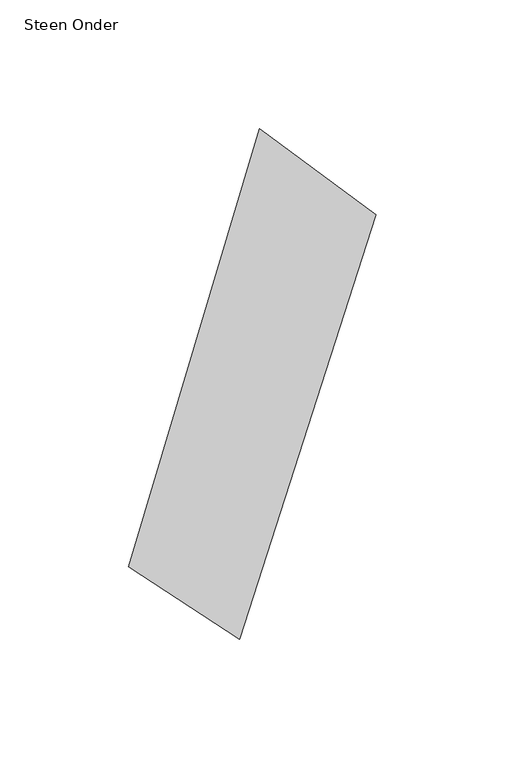
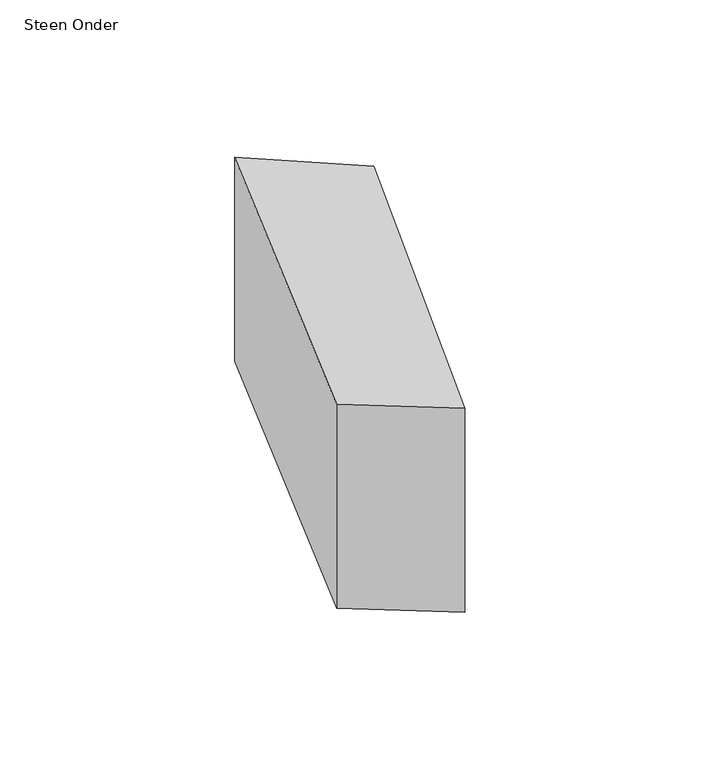
"""IFC4 building model written with IfcOpenShell, lengths in millimetres: proxy geometry, 00_GMA_steen_versie_4 : Steen Onder."""

from ifc_helpers import new_model, si_unit, origin, origin_with_axes, place, context, project, spatial, polyline, outline, extrude, source, transform, mapped, element, save


def steen_onder_082d7394(model_context):
    return source(origin(), model_context, "Body", "SweptSolid", [
        extrude(outline(polyline([(127.1998876, 151.3789965), (74.2256796, -13.1550493), (31.2595891, 14.8619373), (82.1091375, 184.7796986), (127.1998876, 151.3789965)])), origin_with_axes(), (0.0, 0.0, 1.0), 100.0),
    ])


if __name__ == "__main__":
    model = new_model("IFC4")
    model_context = context("Model", 3, world=origin())
    ifc_project = project(units=[si_unit("LENGTHUNIT", "METRE", prefix="MILLI")], contexts=[model_context])
    site = spatial("IfcSite", under=ifc_project)
    building = spatial("IfcBuilding", under=site)
    placement = place(None, origin())
    steen_onder_shape = steen_onder_082d7394(model_context)
    element("IfcBuildingElementProxy", 1, Name="00_GMA_steen_versie_4 : Steen Onder", ObjectType="00_GMA_steen_versie_4 : Steen Onder", at=placement, inside=building, context=model_context, shape_type="MappedRepresentation", body=[
        mapped(steen_onder_shape, transform((0.0, 0.0, 0.0), x_axis=(1.0, 0.0, 0.0), y_axis=(0.0, 1.0, 0.0), z_axis=(0.0, 0.0, 1.0))),
    ])
    save(model, "model.ifc")

# Revit data of these elements
# Type "00_GMA_steen_versie_4 : Steen Onder"
#   StootVoegHalfBoven [instance default] = 5 mm
#   StootVoegHalf [instance default] = 5 mm
#   StootVoegBreedteOnder = 10 mm
#   StootVoegBreedteBoven = 10 mm
#   Steendikte = 100 mm
#   LintVoegOnderHalf = 0 mm
#   LintVoegOnder = 0 mm
#   LintVoegBovenHalf = 5 mm
#   LintVoegBoven = 10 mm
#   materiaal = none
#   MateriaalVoeg = none
#   Default Elevation = 0
